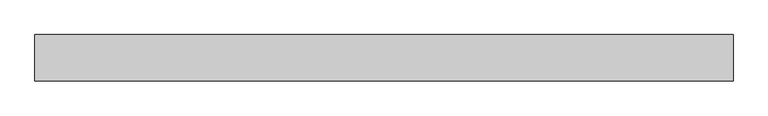
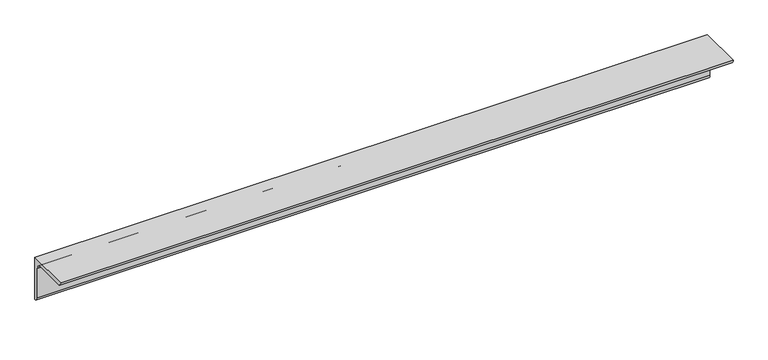
"""IFC4 building model written with IfcOpenShell, lengths in millimetres: beam geometry, 0912_Steel Framing_L-KSD3502 : H_SB_AR_S04_L-100x100x10_KBR2."""

from ifc_helpers import new_model, si_unit, point, frame, frame_2d, origin, place, context, project, spatial, polyline, circle_curve, trimmed, segment, composite_curve, outline, extrude, source, transform, mapped, element, save


def beam_c56ac2bd(model_context):
    return source(origin(), model_context, "Body", "SweptSolid", [
        extrude(outline(composite_curve([segment(polyline([(28.2, 28.2), (28.2, -71.8)]), True, "CONTINUOUS"), segment(trimmed(circle_curve(frame_2d((28.2, -61.8)), 10.0), [point((28.2, -71.8))], [point((18.2, -61.8))], False, "CARTESIAN"), True, "CONTINUOUS"), segment(polyline([(18.2, -61.8), (18.2, 8.2)]), True, "CONTINUOUS"), segment(trimmed(circle_curve(frame_2d((8.2, 8.2)), 10.0), [point((18.2, 8.2))], [point((8.2, 18.2))], True, "CARTESIAN"), True, "CONTINUOUS"), segment(polyline([(8.2, 18.2), (-61.8, 18.2)]), True, "CONTINUOUS"), segment(trimmed(circle_curve(frame_2d((-61.8, 28.2)), 10.0), [point((-61.8, 18.2))], [point((-71.8, 28.2))], False, "CARTESIAN"), True, "CONTINUOUS"), segment(polyline([(-71.8, 28.2), (28.2, 28.2)]), True, "CONTINUOUS")], self_intersect=False)), frame((-835.5368795, 0.0, 0.0), z_axis=(1.0, 0.0, 0.0), x_axis=(0.0, 1.0, 0.0)), (0.0, 0.0, 1.0), 1509.087639),
    ])


if __name__ == "__main__":
    model = new_model("IFC4")
    model_context = context("Model", 3, world=origin())
    ifc_project = project(units=[si_unit("LENGTHUNIT", "METRE", prefix="MILLI")], contexts=[model_context])
    site = spatial("IfcSite", under=ifc_project)
    building = spatial("IfcBuilding", under=site)
    placement = place(None, origin())
    beam_shape = beam_c56ac2bd(model_context)
    element("IfcBeam", 1, ObjectType="0912_Steel Framing_L-KSD3502 : H_SB_AR_S04_L-100x100x10_KBR2", at=placement, inside=building, context=model_context, shape_type="MappedRepresentation", body=[
        mapped(beam_shape, transform((0.0, 0.0, 0.0), x_axis=(1.0, 0.0, 0.0), y_axis=(0.0, 1.0, 0.0), z_axis=(0.0, 0.0, 1.0))),
    ])
    save(model, "model.ifc")

# Revit data of these elements
# Type "0912_Steel Framing_L-KSD3502 : H_SB_AR_S04_L-100x100x10_KBR2"
#   k = 25 mm
#   Perimeter = 0.40 m²/m
#   Nominal Weight = 14.90 kgf/m
#   Length [instance default] = 1000 mm
#   b = 100 mm
#   d = 100 mm
#   t = 10 mm
#   x = 28.2 mm
#   y = 28.2 mm
#   A = 1900.00 m²
#   Structural Material [instance default] = Steel, 45-345
# Element 1 (IfcBeam, "0912_Steel Framing_L-KSD3502 : H_SB_AR_S04_L-100x100x10_KBR2")
#   Structural Material = Steel ASTM A36
#   Materials on its faces: "Steel ASTM A36"
# Materials
#   "Steel, 45-345": class "Metal", colour RGB 189 187 185, transparency 0, Description = "Steel 345 MPa", Cost = 0
#   "Steel ASTM A36": class "Metal", colour RGB 199 199 199, transparency 0, Description = "Structural steel, ASTM A36 Grade B, mill finish", Cost = 0
